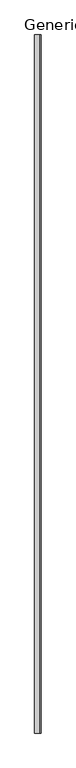
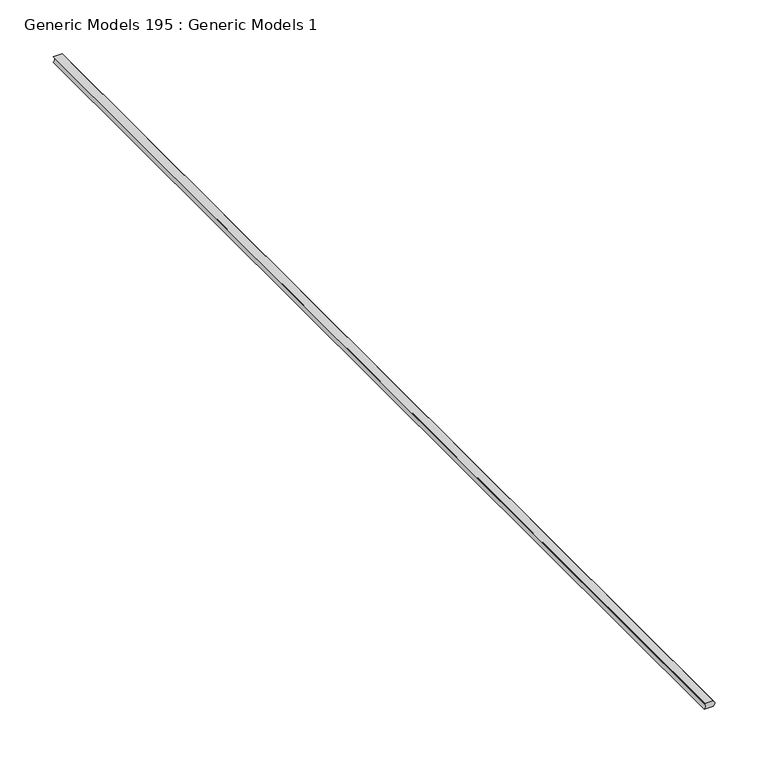
"""IFC4 building model written with IfcOpenShell, lengths in millimetres: proxy geometry, Generic Models 195 : Generic Models 1."""

from ifc_helpers import new_model, si_unit, point, frame, frame_2d, origin, place, context, project, spatial, polyline, circle_curve, trimmed, segment, composite_curve, outline, extrude, source, transform, mapped, element, save


def generic_models_195_generic_models_1_9bd07d6e(model_context):
    return source(origin(), model_context, "Body", "SweptSolid", [
        extrude(outline(composite_curve([segment(polyline([(0.0, 49676.05), (0.0, 49685.575)]), True, "CONTINUOUS"), segment(trimmed(circle_curve(frame_2d((3.175, 49682.6602595)), 4.3100275), [point((0.0, 49685.575))], [point((6.35, 49685.575))], False, "CARTESIAN"), True, "CONTINUOUS"), segment(polyline([(6.35, 49685.575), (6.35, 49676.05)]), True, "CONTINUOUS"), segment(trimmed(circle_curve(frame_2d((3.175, 49673.1352595)), 4.3100275), [point((6.35, 49676.05))], [point((0.0, 49676.05))], True, "CARTESIAN"), True, "CONTINUOUS")], self_intersect=False)), frame((0.0, 0.0, 0.0), z_axis=(0.0, 1.0, 0.0), x_axis=(0.0, 0.0, 1.0)), (0.0, 0.0, 1.0), 1219.2),
    ])


if __name__ == "__main__":
    model = new_model("IFC4")
    model_context = context("Model", 3, world=origin())
    ifc_project = project(units=[si_unit("LENGTHUNIT", "METRE", prefix="MILLI")], contexts=[model_context])
    site = spatial("IfcSite", under=ifc_project)
    building = spatial("IfcBuilding", under=site)
    placement = place(None, origin())
    generic_models_195_generic_models_1_shape = generic_models_195_generic_models_1_9bd07d6e(model_context)
    element("IfcBuildingElementProxy", 1, Name="Generic Models 195 : Generic Models 1", ObjectType="Generic Models 195 : Generic Models 1", at=placement, inside=building, context=model_context, shape_type="MappedRepresentation", body=[
        mapped(generic_models_195_generic_models_1_shape, transform((0.0, 0.0, 0.0), x_axis=(1.0, 0.0, 0.0), y_axis=(0.0, 1.0, 0.0), z_axis=(0.0, 0.0, 1.0))),
    ])
    save(model, "model.ifc")

# Revit data of these elements
# Element 1 (IfcBuildingElementProxy, "Generic Models 195 : Generic Models 1")
#   Materials on its faces: "ACOUSTICAL SEALANT"
# Materials
#   "ACOUSTICAL SEALANT": class "Unassigned", colour RGB 120 120 120, transparency 0, Cost = 0
